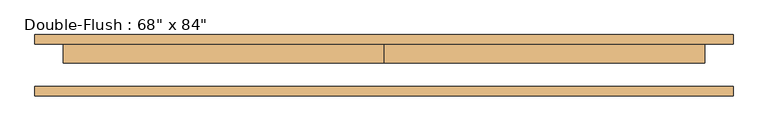
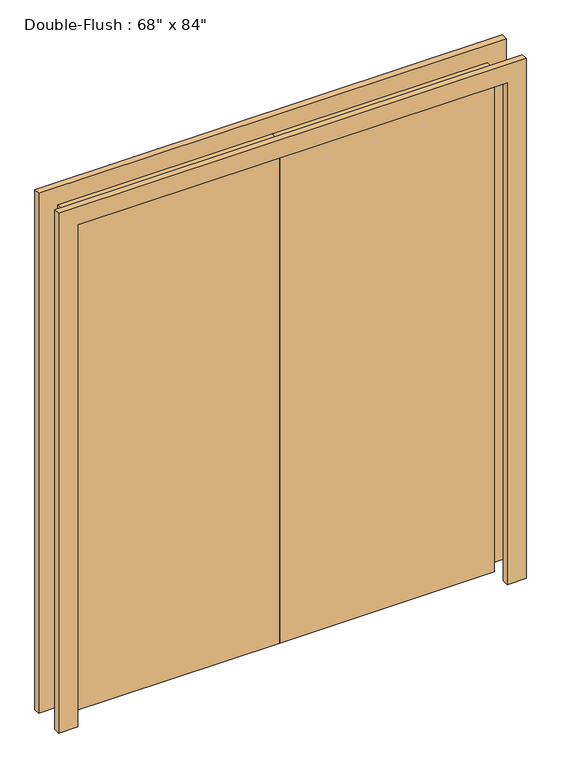
"""IFC4 building model written with IfcOpenShell, lengths in millimetres: door geometry."""

from ifc_helpers import new_model, si_unit, frame, origin, origin_with_axes, place, context, project, spatial, polyline, outline, extrude, source, transform, mapped, element, save


def door_80fcf8b2(model_context):
    return source(origin(), model_context, "Body", "SweptSolid", [
        extrude(outline(polyline([(0.0, 57.15), (863.6, 57.15), (863.6, 6.35), (0.0, 6.35), (0.0, 57.15)])), origin_with_axes(), (0.0, 0.0, 1.0), 2133.6),
        extrude(outline(polyline([(-863.6, 57.15), (0.0, 57.15), (0.0, 6.35), (-863.6, 6.35), (-863.6, 57.15)])), origin_with_axes(), (0.0, 0.0, 1.0), 2133.6),
        extrude(outline(polyline([(2133.6, -863.6), (2133.6, 863.6), (0.0, 863.6), (0.0, 939.8), (2209.8, 939.8), (2209.8, -939.8), (0.0, -939.8), (0.0, -863.6), (2133.6, -863.6)])), frame((0.0, -82.55, 0.0), z_axis=(0.0, 1.0, 0.0), x_axis=(0.0, 0.0, 1.0)), (0.0, 0.0, 1.0), 25.4),
        extrude(outline(polyline([(2133.6, -863.6), (2133.6, 863.6), (0.0, 863.6), (0.0, 939.8), (2209.8, 939.8), (2209.8, -939.8), (0.0, -939.8), (0.0, -863.6), (2133.6, -863.6)])), frame((0.0, 57.15, 0.0), z_axis=(0.0, 1.0, 0.0), x_axis=(0.0, 0.0, 1.0)), (0.0, 0.0, 1.0), 25.4),
    ])


if __name__ == "__main__":
    model = new_model("IFC4")
    model_context = context("Model", 3, world=origin())
    ifc_project = project(units=[si_unit("LENGTHUNIT", "METRE", prefix="MILLI")], contexts=[model_context])
    site = spatial("IfcSite", under=ifc_project)
    building = spatial("IfcBuilding", under=site)
    placement = place(None, origin())
    door_shape = door_80fcf8b2(model_context)
    element("IfcDoor", 1, ObjectType="Double-Flush : 68\" x 84\"", at=placement, inside=building, context=model_context, shape_type="MappedRepresentation", body=[
        mapped(door_shape, transform((0.0, 0.0, 0.0), x_axis=(1.0, 0.0, 0.0), y_axis=(0.0, 1.0, 0.0), z_axis=(0.0, 0.0, 1.0))),
    ])
    save(model, "model.ifc")

# Revit data of these elements
# Type "Double-Flush : 68\" x 84\""
#   Type Mark = "10"
#   Assembly Code = "C1020"
#   Thickness = 0' - 2"
#   Height = 7' - 0"
#   Trim Projection Ext = 0' - 1"
#   Trim Projection Int = 0' - 1"
#   Trim Width = 0' - 3"
#   Width = 5' - 8"
#   Function = 0
#   Door Material = Door - Panel
#   Frame Material = Door - Frame
#   Wall Closure = (empty or 0)
# Element 1 (IfcDoor, "Double-Flush : 68\" x 84\"")
#   Materials on its faces: "Door - Frame", "Door - Panel"
# Materials
#   "Door - Panel": class "Wood", colour RGB 210 159 95, transparency 0
#   "Door - Frame": class "Miscellaneous", colour RGB 118 70 51, transparency 0
